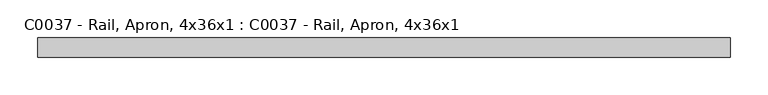
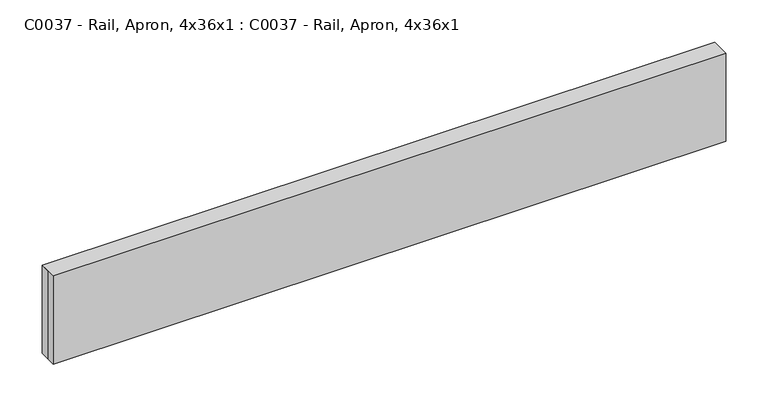
"""IFC4 building model written with IfcOpenShell, lengths in millimetres: proxy geometry, C0037 - Rail, Apron, 4x36x1 : C0037 - Rail, Apron, 4x36x1."""

from ifc_helpers import new_model, si_unit, origin, origin_with_axes, place, context, project, spatial, polyline, outline, extrude, source, transform, mapped, element, save


def c0037_rail_apron_4x36x1_c0037_rail_apron_4x36x1_ed619a96(model_context):
    return source(origin(), model_context, "Body", "SweptSolid", [
        extrude(outline(polyline([(-457.2, 12.7), (457.2, 12.7), (457.2, -12.7), (-457.2, -12.7), (-457.2, 0.0), (-457.2, 12.7)])), origin_with_axes(), (0.0, 0.0, 1.0), 127.0),
        extrude(outline(polyline([(457.2, -12.7), (-457.2, -12.7), (-457.2, 12.7), (457.2, 12.7), (457.2, -12.7)])), origin_with_axes(), (0.0, 0.0, 1.0), 127.0),
    ])


if __name__ == "__main__":
    model = new_model("IFC4")
    model_context = context("Model", 3, world=origin())
    ifc_project = project(units=[si_unit("LENGTHUNIT", "METRE", prefix="MILLI")], contexts=[model_context])
    site = spatial("IfcSite", under=ifc_project)
    building = spatial("IfcBuilding", under=site)
    placement = place(None, origin())
    c0037_rail_apron_4x36x1_c0037_rail_apron_4x36x1_shape = c0037_rail_apron_4x36x1_c0037_rail_apron_4x36x1_ed619a96(model_context)
    element("IfcBuildingElementProxy", 1, Name="C0037 - Rail, Apron, 4x36x1 : C0037 - Rail, Apron, 4x36x1", ObjectType="C0037 - Rail, Apron, 4x36x1 : C0037 - Rail, Apron, 4x36x1", at=placement, inside=building, context=model_context, shape_type="MappedRepresentation", body=[
        mapped(c0037_rail_apron_4x36x1_c0037_rail_apron_4x36x1_shape, transform((0.0, 0.0, 0.0), x_axis=(1.0, 0.0, 0.0), y_axis=(0.0, 1.0, 0.0), z_axis=(0.0, 0.0, 1.0))),
    ])
    save(model, "model.ifc")

# Revit data of these elements
# Type "C0037 - Rail, Apron, 4x36x1 : C0037 - Rail, Apron, 4x36x1"
#   Watts2 = "0"
#   Watts1 = "0"
#   Unit_Issue = "EA"
#   UTIL_6_Misc = "-"
#   UTIL_5_NonMedGas = "-"
#   UTIL_4_MiscGas = "-"
#   UTIL_3_MedGas = "-"
#   UTIL_2_Elec = "-"
#   UTIL_1_WaterDrain = "-"
#   Nomenclature = "Rail, Apron, 4x36x1"
#   NSN = "6530"
#   Location [instance default] = ""
#   JSN = "C0037"
#   Fund_Source_VA = "-"
#   Fund_Source_Navy = "-"
#   Fund_Source_Army = "-"
#   Fund_Source_AF = "-"
#   ELEC_Volts2 = "0"
#   ELEC_Volts1 = "0"
#   ELEC_Phase2 = "0"
#   ELEC_Phase1 = "0"
#   ELEC_HertzSwitch = "0"
#   ELEC_HertzDependent = "0"
#   ELEC_Hertz = "0"
#   ELEC_Amps2 = "0"
#   ELEC_Amps1 = "0"
#   DetailDescription = "Apron rail. Also referred to as an apron front, apron panel, or knee space rail. Used to close in front knee space area and/or provide work surface support between two base cabinets or a base cabinet and wall. Apron rails should be ordered in pairs to provide both front and rear work surface support."
#   CAT_VA = "A"
#   CAT_Navy = "A"
#   CAT_IHS = "-"
#   CAT_Army = "A"
#   CAT_AF = "A"
#   BTUperhour = "0"
#   Weight_IP = 10
#   DIM_Width_IP = 3' - 0"
#   DIM_Height_IP = 0' - 5"
#   DIM_Depth_IP = 0' - 1"
#   Top Panel Material = none
#   Toe Panel Material = none
#   Side Panel Material = none
#   Shelf Panel Material = none
#   Drawer Front Material = none
#   Door Panel Material = none
#   Back Panel Material = none
#   Assembly Code = ""
# Element 1 (IfcBuildingElementProxy, "C0037 - Rail, Apron, 4x36x1 : C0037 - Rail, Apron, 4x36x1")
#   Materials on its faces: "EquipSpace"
# Materials
#   "EquipSpace": class "Unassigned", colour RGB 221 217 195, transparency 0.5
